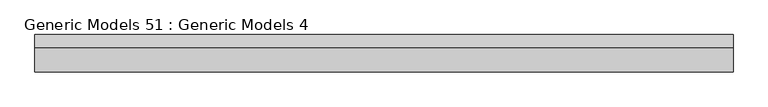
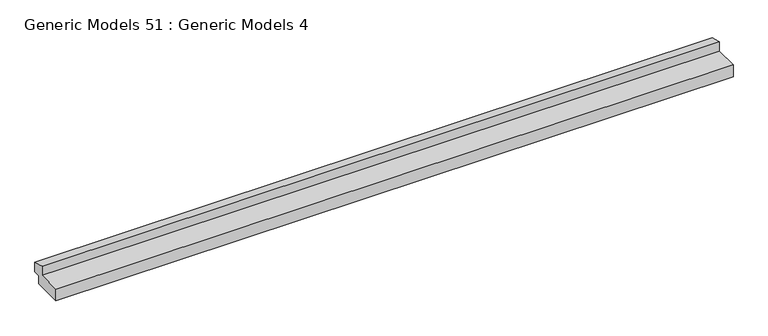
"""IFC4 building model written with IfcOpenShell, lengths in millimetres: proxy geometry, Generic Models 51 : Generic Models 4."""

from ifc_helpers import new_model, si_unit, frame, origin, place, context, project, spatial, polyline, outline, extrude, source, transform, mapped, element, save


def generic_models_51_generic_models_4_c1549c62(model_context):
    return source(origin(), model_context, "Body", "SweptSolid", [
        extrude(outline(polyline([(11233.9215842, 129861.5132036), (11487.9215842, 129798.0132036), (11487.9215842, 129588.5459747), (11348.2215842, 129588.5459747), (11348.2215842, 129410.7459747), (10738.6215842, 129410.7459747), (10738.6215842, 129664.7459747), (11233.9215842, 129664.7459747), (11233.9215842, 129861.5132036)])), frame((-9049.8095964, 0.0, 0.0), z_axis=(1.0, 0.0, 0.0), x_axis=(0.0, 1.0, 0.0)), (0.0, 0.0, 1.0), 13919.2),
    ])


if __name__ == "__main__":
    model = new_model("IFC4")
    model_context = context("Model", 3, world=origin())
    ifc_project = project(units=[si_unit("LENGTHUNIT", "METRE", prefix="MILLI")], contexts=[model_context])
    site = spatial("IfcSite", under=ifc_project)
    building = spatial("IfcBuilding", under=site)
    placement = place(None, origin())
    generic_models_51_generic_models_4_shape = generic_models_51_generic_models_4_c1549c62(model_context)
    element("IfcBuildingElementProxy", 1, Name="Generic Models 51 : Generic Models 4", ObjectType="Generic Models 51 : Generic Models 4", at=placement, inside=building, context=model_context, shape_type="MappedRepresentation", body=[
        mapped(generic_models_51_generic_models_4_shape, transform((0.0, 0.0, 0.0), x_axis=(1.0, 0.0, 0.0), y_axis=(0.0, 1.0, 0.0), z_axis=(0.0, 0.0, 1.0))),
    ])
    save(model, "model.ifc")

# Revit data of these elements
# Element 1 (IfcBuildingElementProxy, "Generic Models 51 : Generic Models 4")
#   Materials on its faces: "_BATT INSUL. (R-FACTOR = R38 MIN) OVER CLASS II VAPOR RETARDER(TOWARD INTERIOR)"
# Materials
#   "_BATT INSUL. (R-FACTOR = R38 MIN) OVER CLASS II VAPOR RETARDER(TOWARD INTERIOR)": class "Generic", colour RGB 227 210 251, transparency 0, Cost = 0
